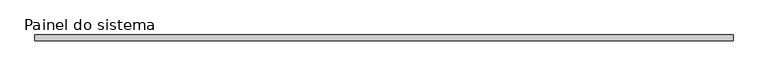
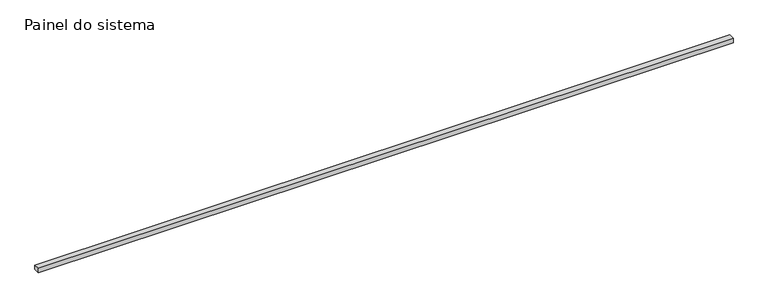
"""IFC4 building model written with IfcOpenShell, lengths in millimetres: plate geometry, Painel do sistema : Envidraçado."""

from ifc_helpers import new_model, si_unit, origin, origin_with_axes, place, context, project, spatial, polyline, outline, extrude, source, transform, mapped, element, save


def painel_do_sistema_42adfd5d(model_context):
    return source(origin(), model_context, "Body", "SweptSolid", [
        extrude(outline(polyline([(1499.9999925, 24.5), (-1499.9999925, 24.5), (-1499.9999925, 49.5), (1499.9999925, 49.5), (1499.9999925, 24.5)])), origin_with_axes(), (0.0, 0.0, 1.0), 20.0931032),
    ])


if __name__ == "__main__":
    model = new_model("IFC4")
    model_context = context("Model", 3, world=origin())
    ifc_project = project(units=[si_unit("LENGTHUNIT", "METRE", prefix="MILLI")], contexts=[model_context])
    site = spatial("IfcSite", under=ifc_project)
    building = spatial("IfcBuilding", under=site)
    placement = place(None, origin())
    painel_do_sistema_shape = painel_do_sistema_42adfd5d(model_context)
    element("IfcPlate", 1, ObjectType="Painel do sistema : Envidraçado", at=placement, inside=building, context=model_context, shape_type="MappedRepresentation", body=[
        mapped(painel_do_sistema_shape, transform((0.0, 0.0, 0.0), x_axis=(1.0, 0.0, 0.0), y_axis=(0.0, 1.0, 0.0), z_axis=(0.0, 0.0, 1.0))),
    ])
    save(model, "model.ifc")

# Revit data of these elements
# Type "Painel do sistema : Envidraçado"
#   Construction Type Id = "GSP4R"
#   Analytic Construction = "Vidraça única Pilkington 1/8 pol"
#   Visual Light Transmittance = 0.9
#   Solar Heat Gain Coefficient = 0.86
#   Heat Transfer Coefficient (U) = 6.7069 W/(m²·K)
# Element 1 (IfcPlate, "Painel do sistema : Envidraçado")
#   Materials on its faces: "Vidro"
# Materials
#   "Vidro": class "Vidro", colour RGB 0 128 192, transparency 0.9, Description = "Vidro de sílica", Cost = 0
